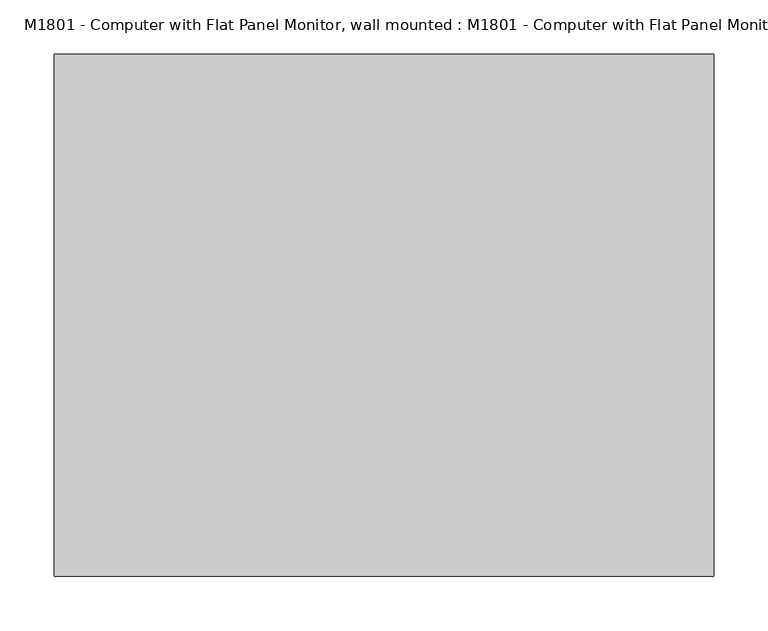
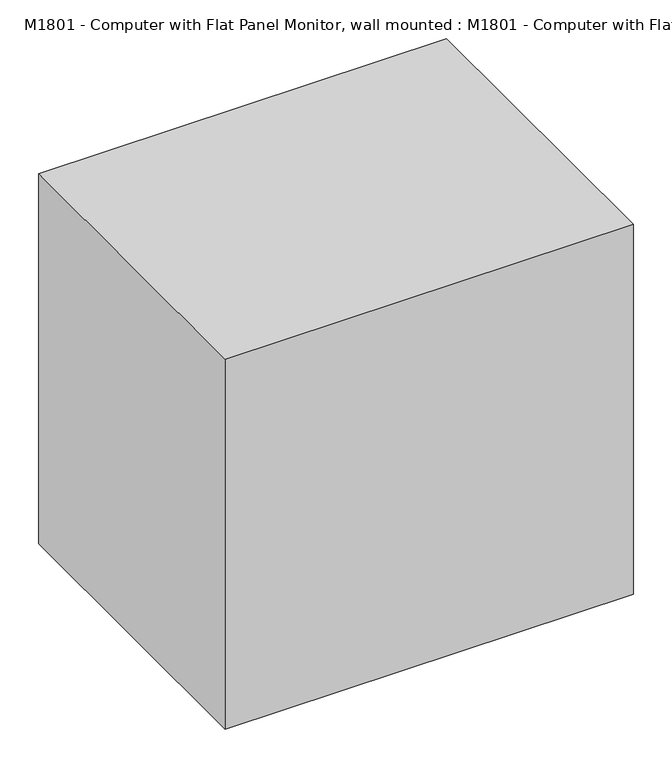
"""IFC4 building model written with IfcOpenShell, lengths in millimetres: proxy geometry, M1801 - Computer with Flat Panel Monitor, wall mounted : M1801 - Computer with Flat Panel Monitor, wall mounted."""

import ifcopenshell
import ifcopenshell.guid

model = None  # the IFC model being written
_history = None  # IfcOwnerHistory: only IFC2X3 demands one
_inside = {}  # id of a spatial element -> (the spatial element, [elements in it])
_under = {}  # id of a project, library or spatial element -> (it, [spatial elements below it])
_declared = {}  # id of a project -> (the project, [libraries it declares])
_typed = {}  # id of a type object -> (the type object, [elements of that type])
_made_of = {}  # id of a material, layer set ... -> (it, [elements and type objects made of it])


def new_model(schema):
    """Start an empty IFC model of exactly this schema.

    Asked for "IFC4X3", IfcOpenShell would pick the latest addendum, in which some entities
    have other attributes; the version numbers below select the first issue.
    IFC2X3 requires an IfcOwnerHistory on every rooted entity: one is made here for all.
    """
    global model, _history
    if schema == "IFC4X3":
        model = ifcopenshell.file(schema_version=(4, 3, 0, 0))
    else:
        model = ifcopenshell.file(schema=schema)
    _inside.clear()
    _under.clear()
    _declared.clear()
    _typed.clear()
    _made_of.clear()
    _history = None
    if model.schema == "IFC2X3":
        org = make("IfcOrganization", Name="unknown")
        user = make(
            "IfcPersonAndOrganization",
            ThePerson=make("IfcPerson", FamilyName="unknown"),
            TheOrganization=org,
        )
        app = make(
            "IfcApplication",
            ApplicationDeveloper=org,
            Version="unknown",
            ApplicationFullName="unknown",
            ApplicationIdentifier="unknown",
        )
        _history = make(
            "IfcOwnerHistory",
            OwningUser=user,
            OwningApplication=app,
            ChangeAction="ADDED",
            CreationDate=0,
        )
    return model


def make(cls, **values):
    """One entity of the class cls with the attributes given. An attribute that is None is left unset."""
    return model.create_entity(
        cls, **{name: value for name, value in values.items() if value is not None}
    )


def rooted(cls, **values):
    """An entity with a GlobalId (a new one), such as an element, a storey or a relation."""
    return make(cls, GlobalId=ifcopenshell.guid.new(), OwnerHistory=_history, **values)


def si_unit(unit_type, name, prefix=None):
    """IfcSIUnit, for example si_unit("LENGTHUNIT", "METRE", prefix="MILLI")."""
    return make("IfcSIUnit", UnitType=unit_type, Prefix=prefix, Name=name)


def assignment(units):
    """IfcUnitAssignment: the units of a project."""
    return None if units is None else make("IfcUnitAssignment", Units=units)


def point(xyz):
    """IfcCartesianPoint."""
    return None if xyz is None else make("IfcCartesianPoint", Coordinates=xyz)


def direction(xyz):
    """IfcDirection."""
    return None if xyz is None else make("IfcDirection", DirectionRatios=xyz)


def frame(location, z_axis=None, x_axis=None):
    """IfcAxis2Placement3D, a coordinate frame: its origin and axes. An axis left out is left unset."""
    return make(
        "IfcAxis2Placement3D",
        Location=point(location),
        Axis=direction(z_axis),
        RefDirection=direction(x_axis),
    )


def origin():
    """The frame at (0, 0, 0) with its axes left unset."""
    return frame((0.0, 0.0, 0.0))


def origin_with_axes():
    """The frame at (0, 0, 0) with the z axis (0, 0, 1) and the x axis (1, 0, 0) written out."""
    return frame((0.0, 0.0, 0.0), z_axis=(0.0, 0.0, 1.0), x_axis=(1.0, 0.0, 0.0))


def place(relative_to, where):
    """IfcLocalPlacement: puts the frame where relative to a parent placement (None: the world)."""
    return make(
        "IfcLocalPlacement", PlacementRelTo=relative_to, RelativePlacement=where
    )


def context(
    kind, dimensions, precision=None, world=None, true_north=None, identifier=None
):
    """IfcGeometricRepresentationContext, for example the 3D "Model" context."""
    return make(
        "IfcGeometricRepresentationContext",
        ContextIdentifier=identifier,
        ContextType=kind,
        CoordinateSpaceDimension=dimensions,
        Precision=precision,
        WorldCoordinateSystem=world,
        TrueNorth=true_north,
    )


def project(units=None, contexts=None):
    """IfcProject with its units and contexts."""
    return rooted(
        "IfcProject",
        Name="project",
        RepresentationContexts=contexts,
        UnitsInContext=assignment(units),
    )


def spatial(cls, under=None, at=None, **own):
    """A site, building, storey or space (cls), placed at a placement, below another one or the project."""
    s = rooted(cls, ObjectPlacement=at, **own)
    if under is not None:
        _under.setdefault(under.id(), (under, []))[1].append(s)
    return s


def polyline(points):
    """IfcPolyline through the points."""
    return make("IfcPolyline", Points=[point(p) for p in points])


def outline(outer, holes=None, kind="AREA"):
    """IfcArbitraryClosedProfileDef: a profile drawn as a closed curve; with holes, ...WithVoids."""
    if holes is None:
        return make("IfcArbitraryClosedProfileDef", ProfileType=kind, OuterCurve=outer)
    return make(
        "IfcArbitraryProfileDefWithVoids",
        ProfileType=kind,
        OuterCurve=outer,
        InnerCurves=holes,
    )


def extrude(swept, where, along, depth):
    """IfcExtrudedAreaSolid: the profile swept, set in the frame where, extruded along a direction by depth."""
    return make(
        "IfcExtrudedAreaSolid",
        SweptArea=swept,
        Position=where,
        ExtrudedDirection=direction(along),
        Depth=depth,
    )


def shape(context_of_items, identifier, shape_type, items):
    """IfcShapeRepresentation: the items that make up one representation, for example the "Body"."""
    return make(
        "IfcShapeRepresentation",
        ContextOfItems=context_of_items,
        RepresentationIdentifier=identifier,
        RepresentationType=shape_type,
        Items=items,
    )


def source(mapping_origin, context_of_items, identifier, shape_type, items):
    """IfcRepresentationMap: a shape defined once, which mapped items show again and again."""
    return make(
        "IfcRepresentationMap",
        MappingOrigin=mapping_origin,
        MappedRepresentation=shape(context_of_items, identifier, shape_type, items),
    )


def transform(
    local_origin,
    x_axis=None,
    y_axis=None,
    z_axis=None,
    scale=None,
    scale2=None,
    scale3=None,
    uniform=True,
):
    """IfcCartesianTransformationOperator3D, or its non-uniform kind. x_axis, y_axis, z_axis: its Axis1, 2, 3."""
    if uniform:
        return make(
            "IfcCartesianTransformationOperator3D",
            Axis1=direction(x_axis),
            Axis2=direction(y_axis),
            LocalOrigin=point(local_origin),
            Scale=scale,
            Axis3=direction(z_axis),
        )
    return make(
        "IfcCartesianTransformationOperator3DnonUniform",
        Axis1=direction(x_axis),
        Axis2=direction(y_axis),
        LocalOrigin=point(local_origin),
        Scale=scale,
        Axis3=direction(z_axis),
        Scale2=scale2,
        Scale3=scale3,
    )


def mapped(mapping_source, mapping_target):
    """IfcMappedItem: shows the shape of a source again, moved by a transform."""
    return make(
        "IfcMappedItem", MappingSource=mapping_source, MappingTarget=mapping_target
    )


def made_of(thing, what):
    """Note that an element or type object is made of a material, layer set ...; save() writes the relation."""
    if what is not None:
        _made_of.setdefault(what.id(), (what, []))[1].append(thing)
    return thing


def element(
    cls,
    number,
    at=None,
    inside=None,
    cuts=None,
    type_object=None,
    material=None,
    context=None,
    identifier="Body",
    shape_type=None,
    held_by="IfcProductDefinitionShape",
    body=None,
    shapes=None,
    **own,
):
    """One element of the class cls, such as IfcWall. Its Tag is "e" and its number.

    at: its placement. inside: the storey or other place that contains it. cuts: it is an
    opening in that element (IfcRelVoidsElement). A single representation is given by context,
    identifier, shape_type and body (its items); several are given by shapes. held_by: the class
    of the entity that holds the representations. save() writes the other relations.
    """
    e = rooted(cls, Tag="e%d" % number, ObjectPlacement=at, **own)
    if body is not None:
        shapes = [shape(context, identifier, shape_type, body)]
    if shapes is not None:
        e.Representation = make(held_by, Representations=shapes)
    if inside is not None:
        _inside.setdefault(inside.id(), (inside, []))[1].append(e)
    if cuts is not None:
        rooted(
            "IfcRelVoidsElement", RelatingBuildingElement=cuts, RelatedOpeningElement=e
        )
    if type_object is not None:
        _typed.setdefault(type_object.id(), (type_object, []))[1].append(e)
    return made_of(e, material)


def aggregate(whole, parts):
    """IfcRelAggregates: a whole, such as a stair, and the parts it consists of."""
    return rooted("IfcRelAggregates", RelatingObject=whole, RelatedObjects=parts)


def save(model, path):
    """Write the relations noted so far, then the file.

    IfcRelAggregates (storeys below a building ...), IfcRelContainedInSpatialStructure (elements
    in a storey), IfcRelDefinesByType, IfcRelAssociatesMaterial and IfcRelDeclares: one each for
    every whole, place, type object, material and project.
    """
    for whole, parts in _under.values():
        aggregate(whole, parts)
    for where, things in _inside.values():
        rooted(
            "IfcRelContainedInSpatialStructure",
            RelatedElements=things,
            RelatingStructure=where,
        )
    for kind, things in _typed.values():
        rooted("IfcRelDefinesByType", RelatedObjects=things, RelatingType=kind)
    for what, things in _made_of.values():
        rooted("IfcRelAssociatesMaterial", RelatedObjects=things, RelatingMaterial=what)
    for by, libraries in _declared.values():
        rooted("IfcRelDeclares", RelatingContext=by, RelatedDefinitions=libraries)
    model.write(path)


def m1801_computer_with_flat_panel_monitor_wall_mounted_m1801_14fd097a(model_context):
    return source(origin(), model_context, "Body", "SweptSolid", [
        extrude(outline(polyline([(431.8, 241.3), (431.8, -241.3), (152.4, -241.3), (152.4, 241.3), (431.8, 241.3)]), holes=[polyline([(419.1, 228.6), (165.1, 228.6), (165.1, -228.6), (419.1, -228.6), (419.1, 228.6)])]), frame((0.0, 82.6343095, 0.0), z_axis=(0.0, 1.0, 0.0), x_axis=(0.0, 0.0, 1.0)), (0.0, 0.0, 1.0), 4.7862024),
        extrude(outline(polyline([(241.3, 87.4205119), (-241.3, 87.4205119), (-241.3, 133.2656905), (241.3, 133.2656905), (241.3, 87.4205119)])), frame((0.0, 0.0, 152.4), z_axis=(0.0, 0.0, 1.0), x_axis=(1.0, 0.0, 0.0)), (0.0, 0.0, 1.0), 279.4),
        extrude(outline(polyline([(304.8, 241.3), (304.8, -241.3), (-304.8, -241.3), (-304.8, 241.3), (304.8, 241.3)])), origin_with_axes(), (0.0, 0.0, 1.0), 584.2),
    ])


if __name__ == "__main__":
    model = new_model("IFC4")
    model_context = context("Model", 3, world=origin())
    ifc_project = project(units=[si_unit("LENGTHUNIT", "METRE", prefix="MILLI")], contexts=[model_context])
    site = spatial("IfcSite", under=ifc_project)
    building = spatial("IfcBuilding", under=site)
    placement = place(None, origin())
    m1801_computer_with_flat_panel_monitor_wall_mounted_m1801_shape = m1801_computer_with_flat_panel_monitor_wall_mounted_m1801_14fd097a(model_context)
    element("IfcBuildingElementProxy", 1, Name="M1801 - Computer with Flat Panel Monitor, wall mounted : M1801 - Computer with Flat Panel Monitor, wall mounted", ObjectType="M1801 - Computer with Flat Panel Monitor, wall mounted : M1801 - Computer with Flat Panel Monitor, wall mounted", at=placement, inside=building, context=model_context, shape_type="MappedRepresentation", body=[
        mapped(m1801_computer_with_flat_panel_monitor_wall_mounted_m1801_shape, transform((0.0, 0.0, 0.0), x_axis=(1.0, 0.0, 0.0), y_axis=(0.0, 1.0, 0.0), z_axis=(0.0, 0.0, 1.0))),
    ])
    save(model, "model.ifc")

# Revit data of these elements
# Type "M1801 - Computer with Flat Panel Monitor, wall mounted : M1801 - Computer with Flat Panel Monitor, wall mounted"
#   Watts2 = "0"
#   Watts1 = "600"
#   Unit_Issue = "EA"
#   UTIL_6_Misc = "-"
#   UTIL_5_NonMedGas = "-"
#   UTIL_4_MiscGas = "-"
#   UTIL_3_MedGas = "-"
#   UTIL_2_Elec = "A"
#   UTIL_1_WaterDrain = "-"
#   Nomenclature = "Computer, Microprocessing, w/Flat Panel Monitor"
#   NSN = "7025"
#   Location [instance default] = ""
#   JSN = "M1801"
#   Fund_Source_VA = "-"
#   Fund_Source_Navy = "-"
#   Fund_Source_Army = "-"
#   Fund_Source_AF = "-"
#   ELEC_Volts2 = "0"
#   ELEC_Volts1 = "120"
#   ELEC_Phase2 = "0"
#   ELEC_Phase1 = "1"
#   ELEC_HertzSwitch = "1"
#   ELEC_HertzDependent = "0"
#   ELEC_Hertz = "60"
#   ELEC_Amps2 = "0"
#   ELEC_Amps1 = "5"
#   DetailDescription = "Desk top microprocessing computer. The unit shall consist of a central processing mini tower, flat panel monitor, keyboard, mouse and speakers. The system shall have the following minimum characteristics: a 2.8 GHz Pentium processor; 512 MB memory; 80GB hard drive; 32/48x CD-ROMDVD combo; 1.44MB network interface card; video 32 MB NVIDIA; a 18 inch flat panel monitor. The computer is used throughout the facility to input, manipulate and retrieve information."
#   CAT_VA = "C"
#   CAT_Navy = "C"
#   CAT_IHS = "-"
#   CAT_Army = "C"
#   CAT_AF = "C"
#   BTUperhour = "0"
#   Weight_IP = 45
#   DIM_Width_IP = 2' - 0"
#   DIM_Height_IP = 1' - 11"
#   DIM_Depth_IP = 1' - 7"
#   Assembly Code = ""
# Element 1 (IfcBuildingElementProxy, "M1801 - Computer with Flat Panel Monitor, wall mounted : M1801 - Computer with Flat Panel Monitor, wall mounted")
#   Location = "DNTS1"
#   Materials on its faces: "EquipSpace"
# Materials
#   "EquipSpace": class "Unassigned", colour RGB 221 217 195, transparency 0.5
